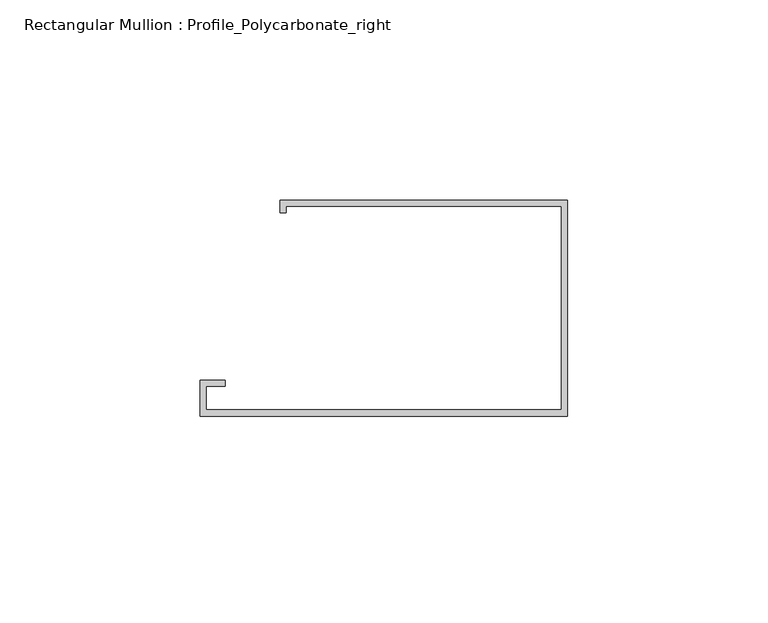
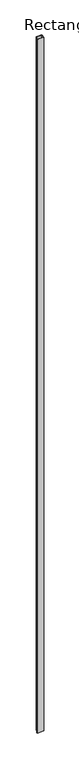
"""IFC4 building model written with IfcOpenShell, lengths in millimetres: member geometry, Rectangular Mullion : Profile_Polycarbonate_right."""

from ifc_helpers import new_model, si_unit, frame, origin, place, context, project, spatial, polyline, outline, extrude, source, transform, mapped, element, save


def rectangular_mullion_profile_polycarbonate_right_3c7db1f8(model_context):
    return source(origin(), model_context, "Body", "SweptSolid", [
        extrude(outline(polyline([(0.0, -28.984575), (-91.9988, -28.984575), (-91.9988, -19.992975), (-85.6488, -19.992975), (-85.6488, -21.580475), (-90.4113, -21.580475), (-90.4113, -27.397075), (-1.5875, -27.397075), (-1.5875, 23.428325), (-70.3961, 23.428325), (-70.3961, 21.840825), (-71.9836, 21.840825), (-71.9836, 25.015825), (0.0, 25.015825), (0.0, -28.984575)])), frame((0.0, 0.0, -9938.791455), z_axis=(0.0, 0.0, 1.0), x_axis=(1.0, 0.0, 0.0)), (0.0, 0.0, 1.0), 9938.791455),
    ])


if __name__ == "__main__":
    model = new_model("IFC4")
    model_context = context("Model", 3, world=origin())
    ifc_project = project(units=[si_unit("LENGTHUNIT", "METRE", prefix="MILLI")], contexts=[model_context])
    site = spatial("IfcSite", under=ifc_project)
    building = spatial("IfcBuilding", under=site)
    placement = place(None, origin())
    rectangular_mullion_profile_polycarbonate_right_shape = rectangular_mullion_profile_polycarbonate_right_3c7db1f8(model_context)
    element("IfcMember", 1, ObjectType="Rectangular Mullion : Profile_Polycarbonate_right", at=placement, inside=building, context=model_context, shape_type="MappedRepresentation", body=[
        mapped(rectangular_mullion_profile_polycarbonate_right_shape, transform((0.0, 0.0, 0.0), x_axis=(1.0, 0.0, 0.0), y_axis=(0.0, 1.0, 0.0), z_axis=(0.0, 0.0, 1.0))),
    ])
    save(model, "model.ifc")

# Revit data of these elements
# Type "Rectangular Mullion : Profile_Polycarbonate_right"
#   built-in parameter 1007322 = 0.177167 (stored number, unit not read)
#   built-in parameter 1007321 = 0 (stored number, unit not read)
#   built-in parameter 1007320 = 0.00520833 (stored number, unit not read)
